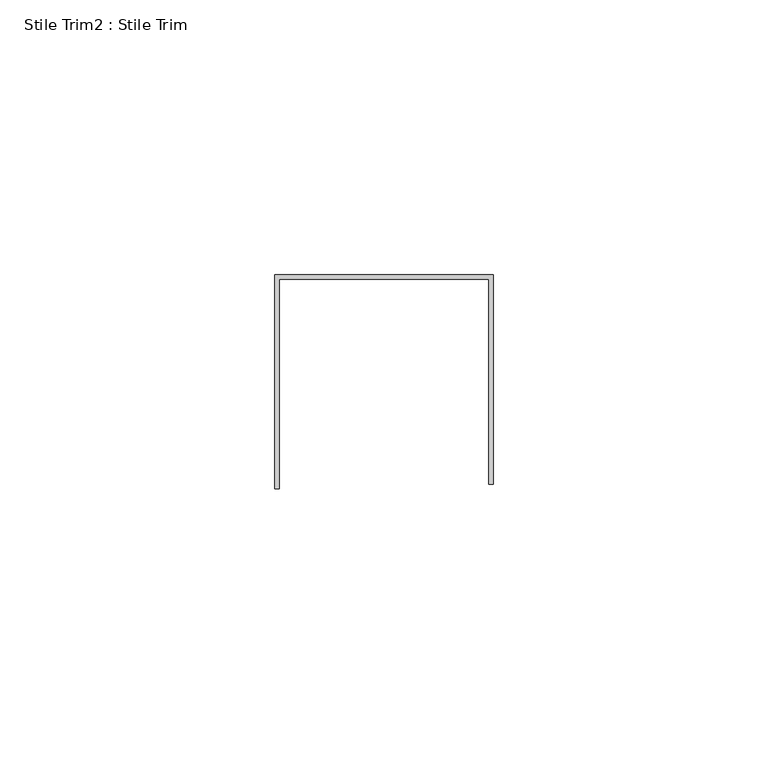
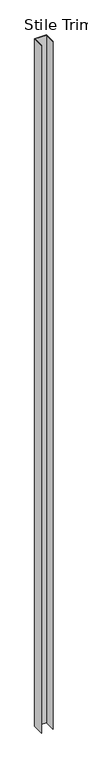
"""IFC4 building model written with IfcOpenShell, lengths in millimetres: proxy geometry, Stile Trim2 : Stile Trim."""

from ifc_helpers import new_model, si_unit, frame, origin, place, context, project, spatial, polyline, outline, extrude, source, transform, mapped, element, save


def stile_trim2_stile_trim_015bedb9(model_context):
    return source(origin(), model_context, "Body", "SweptSolid", [
        extrude(outline(polyline([(587327.0060739, -533994.2789841), (587366.6808739, -533994.2789841), (587366.6808739, -534032.3789841), (587365.8934739, -534032.3789841), (587365.8934739, -533995.0663841), (587327.7934739, -533995.0663841), (587327.7934739, -534033.1663841), (587327.0060739, -534033.1663841), (587327.0060739, -533994.2789841)])), frame((0.0, 0.0, 12.7), z_axis=(0.0, 0.0, 1.0), x_axis=(1.0, 0.0, 0.0)), (0.0, 0.0, 1.0), 2425.7),
    ])


if __name__ == "__main__":
    model = new_model("IFC4")
    model_context = context("Model", 3, world=origin())
    ifc_project = project(units=[si_unit("LENGTHUNIT", "METRE", prefix="MILLI")], contexts=[model_context])
    site = spatial("IfcSite", under=ifc_project)
    building = spatial("IfcBuilding", under=site)
    placement = place(None, origin())
    stile_trim2_stile_trim_shape = stile_trim2_stile_trim_015bedb9(model_context)
    element("IfcBuildingElementProxy", 1, Name="Stile Trim2 : Stile Trim", ObjectType="Stile Trim2 : Stile Trim", at=placement, inside=building, context=model_context, shape_type="MappedRepresentation", body=[
        mapped(stile_trim2_stile_trim_shape, transform((0.0, 0.0, 0.0), x_axis=(1.0, 0.0, 0.0), y_axis=(0.0, 1.0, 0.0), z_axis=(0.0, 0.0, 1.0))),
    ])
    save(model, "model.ifc")

# Revit data of these elements
# Element 1 (IfcBuildingElementProxy, "Stile Trim2 : Stile Trim")
#   Materials on its faces: "EDGE TRIM BY MTL PANEL MFR."
# Materials
#   "EDGE TRIM BY MTL PANEL MFR.": class "Generic", colour RGB 239 242 240, transparency 0, Cost = 0
